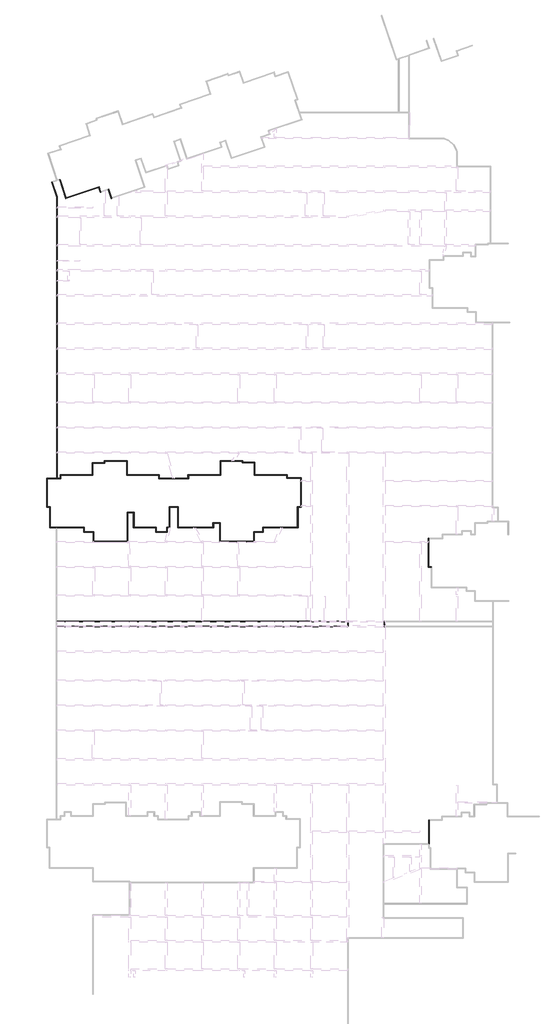
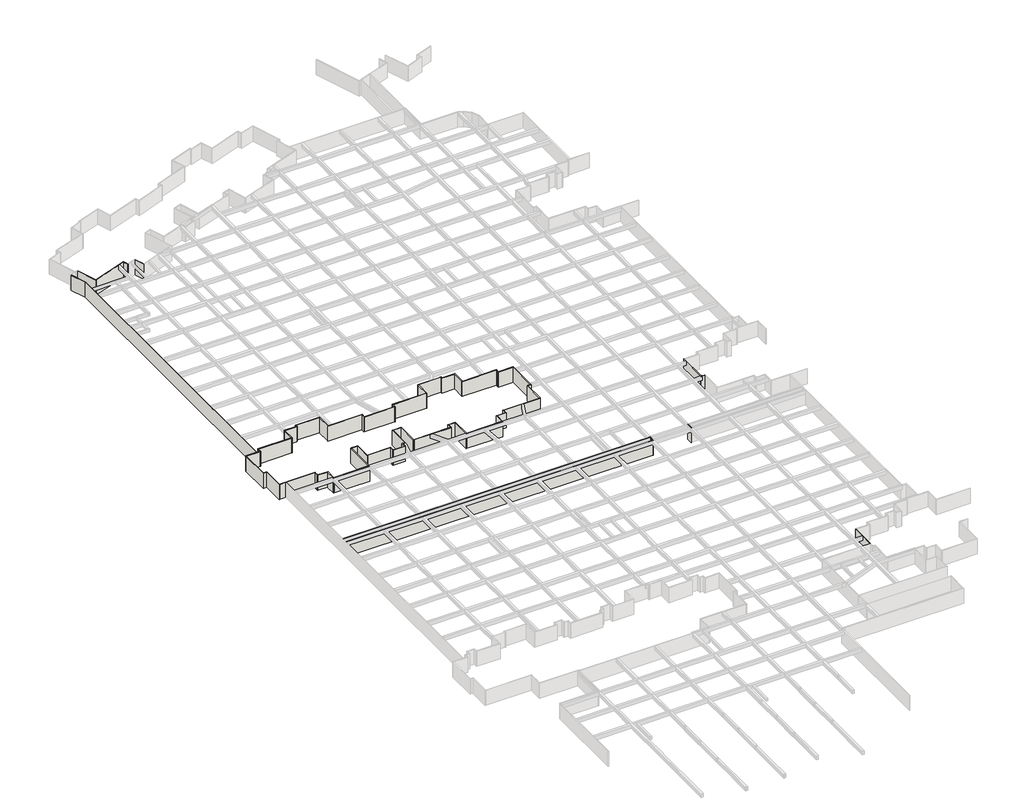
# One storey, part 3 of 14: 65 walls.
"""IFC4 building model written with IfcOpenShell, lengths in millimetres."""

import ifcopenshell
import ifcopenshell.guid

model = None  # the IFC model being written
_history = None  # IfcOwnerHistory: only IFC2X3 demands one
_inside = {}  # id of a spatial element -> (the spatial element, [elements in it])
_under = {}  # id of a project, library or spatial element -> (it, [spatial elements below it])
_declared = {}  # id of a project -> (the project, [libraries it declares])
_typed = {}  # id of a type object -> (the type object, [elements of that type])
_made_of = {}  # id of a material, layer set ... -> (it, [elements and type objects made of it])


def new_model(schema):
    """Start an empty IFC model of exactly this schema.

    Asked for "IFC4X3", IfcOpenShell would pick the latest addendum, in which some entities
    have other attributes; the version numbers below select the first issue.
    IFC2X3 requires an IfcOwnerHistory on every rooted entity: one is made here for all.
    """
    global model, _history
    if schema == "IFC4X3":
        model = ifcopenshell.file(schema_version=(4, 3, 0, 0))
    else:
        model = ifcopenshell.file(schema=schema)
    _inside.clear()
    _under.clear()
    _declared.clear()
    _typed.clear()
    _made_of.clear()
    _history = None
    if model.schema == "IFC2X3":
        org = make("IfcOrganization", Name="unknown")
        user = make(
            "IfcPersonAndOrganization",
            ThePerson=make("IfcPerson", FamilyName="unknown"),
            TheOrganization=org,
        )
        app = make(
            "IfcApplication",
            ApplicationDeveloper=org,
            Version="unknown",
            ApplicationFullName="unknown",
            ApplicationIdentifier="unknown",
        )
        _history = make(
            "IfcOwnerHistory",
            OwningUser=user,
            OwningApplication=app,
            ChangeAction="ADDED",
            CreationDate=0,
        )
    return model


def make(cls, **values):
    """One entity of the class cls with the attributes given. An attribute that is None is left unset."""
    return model.create_entity(
        cls, **{name: value for name, value in values.items() if value is not None}
    )


def rooted(cls, **values):
    """An entity with a GlobalId (a new one), such as an element, a storey or a relation."""
    return make(cls, GlobalId=ifcopenshell.guid.new(), OwnerHistory=_history, **values)


def si_unit(unit_type, name, prefix=None):
    """IfcSIUnit, for example si_unit("LENGTHUNIT", "METRE", prefix="MILLI")."""
    return make("IfcSIUnit", UnitType=unit_type, Prefix=prefix, Name=name)


def assignment(units):
    """IfcUnitAssignment: the units of a project."""
    return None if units is None else make("IfcUnitAssignment", Units=units)


def point(xyz):
    """IfcCartesianPoint."""
    return None if xyz is None else make("IfcCartesianPoint", Coordinates=xyz)


def direction(xyz):
    """IfcDirection."""
    return None if xyz is None else make("IfcDirection", DirectionRatios=xyz)


def frame(location, z_axis=None, x_axis=None):
    """IfcAxis2Placement3D, a coordinate frame: its origin and axes. An axis left out is left unset."""
    return make(
        "IfcAxis2Placement3D",
        Location=point(location),
        Axis=direction(z_axis),
        RefDirection=direction(x_axis),
    )


def origin():
    """The frame at (0, 0, 0) with its axes left unset."""
    return frame((0.0, 0.0, 0.0))


def origin_with_axes():
    """The frame at (0, 0, 0) with the z axis (0, 0, 1) and the x axis (1, 0, 0) written out."""
    return frame((0.0, 0.0, 0.0), z_axis=(0.0, 0.0, 1.0), x_axis=(1.0, 0.0, 0.0))


def place(relative_to, where):
    """IfcLocalPlacement: puts the frame where relative to a parent placement (None: the world)."""
    return make(
        "IfcLocalPlacement", PlacementRelTo=relative_to, RelativePlacement=where
    )


def context(
    kind, dimensions, precision=None, world=None, true_north=None, identifier=None
):
    """IfcGeometricRepresentationContext, for example the 3D "Model" context."""
    return make(
        "IfcGeometricRepresentationContext",
        ContextIdentifier=identifier,
        ContextType=kind,
        CoordinateSpaceDimension=dimensions,
        Precision=precision,
        WorldCoordinateSystem=world,
        TrueNorth=true_north,
    )


def project(units=None, contexts=None):
    """IfcProject with its units and contexts."""
    return rooted(
        "IfcProject",
        Name="project",
        RepresentationContexts=contexts,
        UnitsInContext=assignment(units),
    )


def spatial(cls, under=None, at=None, **own):
    """A site, building, storey or space (cls), placed at a placement, below another one or the project."""
    s = rooted(cls, ObjectPlacement=at, **own)
    if under is not None:
        _under.setdefault(under.id(), (under, []))[1].append(s)
    return s


def polyline(points):
    """IfcPolyline through the points."""
    return make("IfcPolyline", Points=[point(p) for p in points])


def outline(outer, holes=None, kind="AREA"):
    """IfcArbitraryClosedProfileDef: a profile drawn as a closed curve; with holes, ...WithVoids."""
    if holes is None:
        return make("IfcArbitraryClosedProfileDef", ProfileType=kind, OuterCurve=outer)
    return make(
        "IfcArbitraryProfileDefWithVoids",
        ProfileType=kind,
        OuterCurve=outer,
        InnerCurves=holes,
    )


def extrude(swept, where, along, depth):
    """IfcExtrudedAreaSolid: the profile swept, set in the frame where, extruded along a direction by depth."""
    return make(
        "IfcExtrudedAreaSolid",
        SweptArea=swept,
        Position=where,
        ExtrudedDirection=direction(along),
        Depth=depth,
    )


def faces_of(points, faces, orient=None, outer=None):
    """IfcFace entities. A face is a list of loops; a loop is a list of indices into points, from 0.

    orient and outer hold one flag for each loop. By default every Orientation is true, the
    first loop of a face is its IfcFaceOuterBound and the others are IfcFaceBound.
    """
    made = []
    for i, loops in enumerate(faces):
        bounds = []
        for j, loop in enumerate(loops):
            is_outer = j == 0 if outer is None else outer[i][j]
            bounds.append(
                make(
                    "IfcFaceOuterBound" if is_outer else "IfcFaceBound",
                    Bound=make("IfcPolyLoop", Polygon=[points[k] for k in loop]),
                    Orientation=True if orient is None else orient[i][j],
                )
            )
        made.append(make("IfcFace", Bounds=bounds))
    return made


def faceted_brep(points, faces, orient=None, outer=None, voids=None):
    """IfcFacetedBrep: a solid bounded by flat faces; with voids (closed shells), ...WithVoids."""
    shared = [point(p) for p in points]
    hull = make("IfcClosedShell", CfsFaces=faces_of(shared, faces, orient, outer))
    if voids is None:
        return make("IfcFacetedBrep", Outer=hull)
    return make(
        "IfcFacetedBrepWithVoids",
        Outer=hull,
        Voids=[
            make(cls, CfsFaces=faces_of(shared, fs, o, b)) for cls, fs, o, b in voids
        ],
    )


def shape(context_of_items, identifier, shape_type, items):
    """IfcShapeRepresentation: the items that make up one representation, for example the "Body"."""
    return make(
        "IfcShapeRepresentation",
        ContextOfItems=context_of_items,
        RepresentationIdentifier=identifier,
        RepresentationType=shape_type,
        Items=items,
    )


def made_of(thing, what):
    """Note that an element or type object is made of a material, layer set ...; save() writes the relation."""
    if what is not None:
        _made_of.setdefault(what.id(), (what, []))[1].append(thing)
    return thing


def element(
    cls,
    number,
    at=None,
    inside=None,
    cuts=None,
    type_object=None,
    material=None,
    context=None,
    identifier="Body",
    shape_type=None,
    held_by="IfcProductDefinitionShape",
    body=None,
    shapes=None,
    **own,
):
    """One element of the class cls, such as IfcWall. Its Tag is "e" and its number.

    at: its placement. inside: the storey or other place that contains it. cuts: it is an
    opening in that element (IfcRelVoidsElement). A single representation is given by context,
    identifier, shape_type and body (its items); several are given by shapes. held_by: the class
    of the entity that holds the representations. save() writes the other relations.
    """
    e = rooted(cls, Tag="e%d" % number, ObjectPlacement=at, **own)
    if body is not None:
        shapes = [shape(context, identifier, shape_type, body)]
    if shapes is not None:
        e.Representation = make(held_by, Representations=shapes)
    if inside is not None:
        _inside.setdefault(inside.id(), (inside, []))[1].append(e)
    if cuts is not None:
        rooted(
            "IfcRelVoidsElement", RelatingBuildingElement=cuts, RelatedOpeningElement=e
        )
    if type_object is not None:
        _typed.setdefault(type_object.id(), (type_object, []))[1].append(e)
    return made_of(e, material)


def aggregate(whole, parts):
    """IfcRelAggregates: a whole, such as a stair, and the parts it consists of."""
    return rooted("IfcRelAggregates", RelatingObject=whole, RelatedObjects=parts)


def save(model, path):
    """Write the relations noted so far, then the file.

    IfcRelAggregates (storeys below a building ...), IfcRelContainedInSpatialStructure (elements
    in a storey), IfcRelDefinesByType, IfcRelAssociatesMaterial and IfcRelDeclares: one each for
    every whole, place, type object, material and project.
    """
    for whole, parts in _under.values():
        aggregate(whole, parts)
    for where, things in _inside.values():
        rooted(
            "IfcRelContainedInSpatialStructure",
            RelatedElements=things,
            RelatingStructure=where,
        )
    for kind, things in _typed.values():
        rooted("IfcRelDefinesByType", RelatedObjects=things, RelatingType=kind)
    for what, things in _made_of.values():
        rooted("IfcRelAssociatesMaterial", RelatedObjects=things, RelatingMaterial=what)
    for by, libraries in _declared.values():
        rooted("IfcRelDeclares", RelatingContext=by, RelatedDefinitions=libraries)
    model.write(path)


model = new_model("IFC4")

# Units and contexts
model_context = context("Model", 3, world=origin())
ifc_project = project(units=[si_unit("LENGTHUNIT", "METRE", prefix="MILLI")], contexts=[model_context])

# Site, building, storey
site = spatial("IfcSite", under=ifc_project)
building = spatial("IfcBuilding", under=site)
storey = spatial("IfcBuildingStorey", under=building, Name="户型图", Elevation=0.0)

# Walls
placement = place(None, origin())
element("IfcWall", 1, ObjectType="所有墙体", at=placement, inside=storey, context=model_context, shape_type="Brep", body=[
    faceted_brep([(-593530.5298151, -30931.4697976, 0.0), (-592123.7332007, -35098.9851149, 0.0), (-592123.7332007, -35098.9851149, 3300.0), (-593530.5298151, -30931.4697976, 3300.0), (-593416.7566971, -30893.3157103, 0.0), (-593416.7566971, -30893.3157103, 3300.0), (-592048.3399682, -34947.133881, 3300.0), (-592009.9600827, -35060.8310276, 3300.0), (-592009.9600827, -35060.8310276, 0.0), (-592048.3399682, -34947.133881, 0.0)], [[[0, 1, 2, 3]], [[4, 5, 6, 7, 8, 9]], [[1, 0, 4, 9, 8]], [[3, 2, 7, 6, 5]], [[0, 3, 5, 4]], [[2, 1, 8, 7]]]),
])
element("IfcWall", 2, ObjectType="所有墙体", at=placement, inside=storey, context=model_context, shape_type="Brep", body=[
    faceted_brep([(-592009.9600827, -35060.8310276, 0.0), (-584918.2294187, -32682.6021846, 0.0), (-584804.4565249, -32644.4481725, 0.0), (-584804.4565249, -32644.4481725, 3300.0), (-584918.2294187, -32682.6021846, 3300.0), (-592009.9600827, -35060.8310276, 3300.0), (-592048.3399682, -34947.133881, 0.0), (-592048.3399682, -34947.133881, 3300.0), (-584842.610537, -32530.6752787, 3300.0), (-584842.610537, -32530.6752787, 0.0)], [[[0, 1, 2, 3, 4, 5]], [[6, 7, 8, 9]], [[2, 1, 0, 6, 9]], [[5, 4, 3, 8, 7]], [[0, 5, 7, 6]], [[3, 2, 9, 8]]]),
])
element("IfcWall", 3, ObjectType="所有墙体", at=placement, inside=storey, context=model_context, shape_type="Brep", body=[
    faceted_brep([(-584918.2294187, -32682.6021846, 0.0), (-584573.2781333, -33711.2254879, 0.0), (-584573.2781333, -33711.2254879, 3300.0), (-584918.2294187, -32682.6021846, 3300.0), (-584804.4565249, -32644.4481725, 0.0), (-584804.4565249, -32644.4481725, 3300.0), (-584497.735074, -33559.0724844, 3300.0), (-584459.5809867, -33672.8456024, 3300.0), (-584459.5809867, -33672.8456024, 0.0), (-584497.735074, -33559.0724844, 0.0)], [[[0, 1, 2, 3]], [[4, 5, 6, 7, 8, 9]], [[1, 0, 4, 9, 8]], [[3, 2, 7, 6, 5]], [[0, 3, 5, 4]], [[2, 1, 8, 7]]]),
])
element("IfcWall", 4, ObjectType="所有墙体", at=placement, inside=storey, context=model_context, shape_type="Brep", body=[
    faceted_brep([(-582772.9638867, -33103.5070288, 0.0), (-582101.3172132, -35093.2031729, 0.0), (-582101.3172132, -35093.2031729, 3300.0), (-582772.9638867, -33103.5070288, 3300.0), (-582659.2669642, -33065.1272189, 0.0), (-582659.2669642, -33065.1272189, 3300.0), (-582026.0001006, -34941.1264405, 3300.0), (-581987.6202907, -35054.823363, 3300.0), (-581987.6202907, -35054.823363, 0.0), (-582026.0001006, -34941.1264405, 0.0)], [[[0, 1, 2, 3]], [[4, 5, 6, 7, 8, 9]], [[1, 0, 4, 9, 8]], [[3, 2, 7, 6, 5]], [[0, 3, 5, 4]], [[2, 1, 8, 7]]]),
])
element("IfcWall", 5, ObjectType="所有墙体", at=placement, inside=storey, context=model_context, shape_type="SweptSolid", body=[
    extrude(outline(polyline([(-594139.2557706, -34756.12632), (-595236.3254494, -31506.1507065), (-595122.6285269, -31467.7708966), (-594019.2557706, -34736.418841), (-594139.2557706, -34756.12632)])), origin_with_axes(), (0.0, 0.0, 1.0), 3300.0),
])
element("IfcWall", 6, ObjectType="所有墙体", at=placement, inside=storey, context=model_context, shape_type="SweptSolid", body=[
    extrude(outline(polyline([(-594139.2557706, -96686.2725805), (-594139.2557706, -34756.12632), (-594019.2557706, -34736.418841), (-594019.2557706, -96686.2725805), (-594139.2557706, -96686.2725805)])), origin_with_axes(), (0.0, 0.0, 1.0), 3300.0),
])
element("IfcWall", 7, ObjectType="所有墙体", at=placement, inside=storey, context=model_context, shape_type="Brep", body=[
    faceted_brep([(-593387.5937633, -96686.2725805, 0.0), (-594019.2557706, -96686.2725805, 0.0), (-594139.2557706, -96686.2725805, 0.0), (-596357.5937917, -96686.2725805, 0.0), (-596357.5937917, -96686.2725805, 3300.0), (-594139.2557706, -96686.2725805, 3300.0), (-594019.2557706, -96686.2725805, 3300.0), (-593387.5937633, -96686.2725805, 3300.0), (-593387.5937633, -96806.2725805, 0.0), (-593387.5937633, -96806.2725805, 3300.0), (-596237.5937917, -96806.2725805, 3300.0), (-596357.5937917, -96806.2725805, 3300.0), (-596357.5937917, -96806.2725805, 0.0), (-596237.5937917, -96806.2725805, 0.0)], [[[0, 1, 2, 3, 4, 5, 6, 7]], [[8, 9, 10, 11, 12, 13]], [[3, 2, 1, 0, 8, 13, 12]], [[7, 6, 5, 4, 11, 10, 9]], [[4, 3, 12, 11]], [[0, 7, 9, 8]]]),
])
element("IfcWall", 8, ObjectType="所有墙体", at=placement, inside=storey, context=model_context, shape_type="Brep", body=[
    faceted_brep([(-596357.5937917, -96806.2725805, 0.0), (-596357.5937917, -103075.8355436, 0.0), (-596357.5937917, -103075.8355436, 3300.0), (-596357.5937917, -96806.2725805, 3300.0), (-596237.5937917, -96806.2725805, 0.0), (-596237.5937917, -96806.2725805, 3300.0), (-596237.5937917, -102955.8355436, 3300.0), (-596237.5937917, -103075.8355436, 3300.0), (-596237.5937917, -103075.8355436, 0.0), (-596237.5937917, -102955.8355436, 0.0)], [[[0, 1, 2, 3]], [[4, 5, 6, 7, 8, 9]], [[1, 0, 4, 9, 8]], [[3, 2, 7, 6, 5]], [[0, 3, 5, 4]], [[2, 1, 8, 7]]]),
])
element("IfcWall", 9, ObjectType="所有墙体", at=placement, inside=storey, context=model_context, shape_type="Brep", body=[
    faceted_brep([(-596237.5937917, -103075.8355436, 0.0), (-595657.5937933, -103075.8355436, 0.0), (-595537.5937933, -103075.8355436, 0.0), (-595537.5937933, -103075.8355436, 3300.0), (-595657.5937933, -103075.8355436, 3300.0), (-596237.5937917, -103075.8355436, 3300.0), (-596237.5937917, -102955.8355436, 0.0), (-596237.5937917, -102955.8355436, 3300.0), (-595537.5937933, -102955.8355436, 3300.0), (-595537.5937933, -102955.8355436, 0.0)], [[[0, 1, 2, 3, 4, 5]], [[6, 7, 8, 9]], [[2, 1, 0, 6, 9]], [[5, 4, 3, 8, 7]], [[0, 5, 7, 6]], [[3, 2, 9, 8]]]),
])
element("IfcWall", 10, ObjectType="所有墙体", at=placement, inside=storey, context=model_context, shape_type="Brep", body=[
    faceted_brep([(-595657.5937933, -103075.8355436, 0.0), (-595657.5937933, -107575.8355437, 0.0), (-595657.5937933, -107575.8355437, 3300.0), (-595657.5937933, -103075.8355436, 3300.0), (-595537.5937933, -103075.8355436, 0.0), (-595537.5937933, -103075.8355436, 3300.0), (-595537.5937933, -107455.8355437, 3300.0), (-595537.5937933, -107575.8355437, 3300.0), (-595537.5937933, -107575.8355437, 0.0), (-595537.5937933, -107455.8355437, 0.0)], [[[0, 1, 2, 3]], [[4, 5, 6, 7, 8, 9]], [[1, 0, 4, 9, 8]], [[3, 2, 7, 6, 5]], [[0, 3, 5, 4]], [[2, 1, 8, 7]]]),
])
element("IfcWall", 11, ObjectType="所有墙体", at=placement, inside=storey, context=model_context, shape_type="Brep", body=[
    faceted_brep([(-595537.5937933, -107575.8355437, 0.0), (-594257.5937933, -107575.8355437, 0.0), (-594137.5937933, -107575.8355437, 0.0), (-588182.5937843, -107575.8355437, 0.0), (-588062.5937843, -107575.8355437, 0.0), (-588062.5937843, -107575.8355437, 3300.0), (-588182.5937843, -107575.8355437, 3300.0), (-594137.5937933, -107575.8355437, 3300.0), (-594257.5937933, -107575.8355437, 3300.0), (-595537.5937933, -107575.8355437, 3300.0), (-595537.5937933, -107455.8355437, 0.0), (-595537.5937933, -107455.8355437, 3300.0), (-588062.5937843, -107455.8355437, 3300.0), (-588062.5937843, -107455.8355437, 0.0)], [[[0, 1, 2, 3, 4, 5, 6, 7, 8, 9]], [[10, 11, 12, 13]], [[4, 3, 2, 1, 0, 10, 13]], [[9, 8, 7, 6, 5, 12, 11]], [[0, 9, 11, 10]], [[5, 4, 13, 12]]]),
])
element("IfcWall", 12, ObjectType="所有墙体", at=placement, inside=storey, context=model_context, shape_type="Brep", body=[
    faceted_brep([(-588182.5937843, -107575.8355437, 0.0), (-588182.5937843, -108525.8355399, 0.0), (-588182.5937843, -108525.8355399, 3300.0), (-588182.5937843, -107575.8355437, 3300.0), (-588062.5937843, -107575.8355437, 0.0), (-588062.5937843, -107575.8355437, 3300.0), (-588062.5937843, -108405.8355399, 3300.0), (-588062.5937843, -108525.8355399, 3300.0), (-588062.5937843, -108525.8355399, 0.0), (-588062.5937843, -108405.8355399, 0.0)], [[[0, 1, 2, 3]], [[4, 5, 6, 7, 8, 9]], [[1, 0, 4, 9, 8]], [[3, 2, 7, 6, 5]], [[0, 3, 5, 4]], [[2, 1, 8, 7]]]),
])
element("IfcWall", 13, ObjectType="所有墙体", at=placement, inside=storey, context=model_context, shape_type="Brep", body=[
    faceted_brep([(-588062.5937843, -108525.8355399, 0.0), (-586077.6529954, -108525.8355399, 0.0), (-585957.6529954, -108525.8355399, 0.0), (-585957.6529954, -108525.8355399, 3300.0), (-586077.6529954, -108525.8355399, 3300.0), (-588062.5937843, -108525.8355399, 3300.0), (-588062.5937843, -108405.8355399, 0.0), (-588062.5937843, -108405.8355399, 3300.0), (-585957.6529954, -108405.8355399, 3300.0), (-585957.6529954, -108405.8355399, 0.0)], [[[0, 1, 2, 3, 4, 5]], [[6, 7, 8, 9]], [[2, 1, 0, 6, 9]], [[5, 4, 3, 8, 7]], [[0, 5, 7, 6]], [[3, 2, 9, 8]]]),
])
element("IfcWall", 14, ObjectType="所有墙体", at=placement, inside=storey, context=model_context, shape_type="Brep", body=[
    faceted_brep([(-586077.6529954, -108525.8355399, 0.0), (-586077.6529954, -110675.8355352, 0.0), (-586077.6529954, -110675.8355352, 2500.0), (-586077.6529954, -110675.8355352, 3300.0), (-586077.6529954, -110459.4327531, 3300.0), (-586077.6529954, -108525.8355399, 3300.0), (-585957.6529954, -108525.8355399, 0.0), (-585957.6529954, -108525.8355399, 3300.0), (-585957.6529954, -110459.4327531, 3300.0), (-585957.6529954, -110555.8355352, 3300.0), (-585957.6529954, -110675.8355352, 3300.0), (-585957.6529954, -110675.8355352, 0.0), (-585957.6529954, -110555.8355352, 0.0)], [[[0, 1, 2, 3, 4, 5]], [[6, 7, 8, 9, 10, 11, 12]], [[1, 0, 6, 12, 11]], [[5, 4, 3, 10, 9, 8, 7]], [[0, 5, 7, 6]], [[3, 2, 1, 11, 10]]]),
])
element("IfcWall", 15, ObjectType="所有墙体", at=placement, inside=storey, context=model_context, shape_type="Brep", body=[
    faceted_brep([(-585957.6529954, -110675.8355352, 0.0), (-578537.5937894, -110675.8355352, 0.0), (-578537.5937894, -110675.8355352, 2500.0), (-578537.5937894, -110675.8355352, 3300.0), (-585957.6529954, -110675.8355352, 3300.0), (-585957.6529954, -110555.8355352, 0.0), (-585957.6529954, -110555.8355352, 2500.0), (-585957.6529954, -110555.8355352, 3300.0), (-578657.5937894, -110555.8355352, 3300.0), (-578537.5937894, -110555.8355352, 3300.0), (-578537.5937894, -110555.8355352, 0.0), (-578657.5937894, -110555.8355352, 0.0)], [[[0, 1, 2, 3, 4]], [[5, 6, 7, 8, 9, 10, 11]], [[1, 0, 5, 11, 10]], [[4, 3, 9, 8, 7]], [[0, 4, 7, 6, 5]], [[3, 2, 1, 10, 9]]]),
])
element("IfcWall", 16, ObjectType="所有墙体", at=placement, inside=storey, context=model_context, shape_type="Brep", body=[
    faceted_brep([(-578537.5937894, -110555.8355352, 0.0), (-578537.5937894, -104200.8355452, 0.0), (-578537.5937894, -104080.8355452, 0.0), (-578537.5937894, -104080.8355452, 3300.0), (-578537.5937894, -104200.8355452, 3300.0), (-578537.5937894, -110459.4327531, 3300.0), (-578537.5937894, -110555.8355352, 3300.0), (-578657.5937894, -110555.8355352, 0.0), (-578657.5937894, -110555.8355352, 2500.0), (-578657.5937894, -110555.8355352, 3300.0), (-578657.5937894, -110459.4327531, 3300.0), (-578657.5937894, -104080.8355452, 3300.0), (-578657.5937894, -104080.8355452, 0.0)], [[[0, 1, 2, 3, 4, 5, 6]], [[7, 8, 9, 10, 11, 12]], [[2, 1, 0, 7, 12]], [[6, 5, 4, 3, 11, 10, 9]], [[0, 6, 9, 8, 7]], [[3, 2, 12, 11]]]),
])
element("IfcWall", 17, ObjectType="所有墙体", at=placement, inside=storey, context=model_context, shape_type="Brep", body=[
    faceted_brep([(-578537.5937894, -104200.8355452, 0.0), (-577257.5937775, -104200.8355452, 0.0), (-577137.5937775, -104200.8355452, 0.0), (-577137.5937775, -104200.8355452, 3300.0), (-577257.5937775, -104200.8355452, 3300.0), (-578537.5937894, -104200.8355452, 3300.0), (-578537.5937894, -104080.8355452, 0.0), (-578537.5937894, -104080.8355452, 3300.0), (-577137.5937775, -104080.8355452, 3300.0), (-577137.5937775, -104080.8355452, 0.0)], [[[0, 1, 2, 3, 4, 5]], [[6, 7, 8, 9]], [[2, 1, 0, 6, 9]], [[5, 4, 3, 8, 7]], [[0, 5, 7, 6]], [[3, 2, 9, 8]]]),
])
element("IfcWall", 18, ObjectType="所有墙体", at=placement, inside=storey, context=model_context, shape_type="Brep", body=[
    faceted_brep([(-577257.5937775, -104200.8355452, 0.0), (-577257.5937775, -107575.8355437, 0.0), (-577257.5937775, -107575.8355437, 3300.0), (-577257.5937775, -104200.8355452, 3300.0), (-577137.5937775, -104200.8355452, 0.0), (-577137.5937775, -104200.8355452, 3300.0), (-577137.5937775, -107455.8355437, 3300.0), (-577137.5937775, -107575.8355437, 3300.0), (-577137.5937775, -107575.8355437, 0.0), (-577137.5937775, -107455.8355437, 0.0)], [[[0, 1, 2, 3]], [[4, 5, 6, 7, 8, 9]], [[1, 0, 4, 9, 8]], [[3, 2, 7, 6, 5]], [[0, 3, 5, 4]], [[2, 1, 8, 7]]]),
])
element("IfcWall", 19, ObjectType="所有墙体", at=placement, inside=storey, context=model_context, shape_type="Brep", body=[
    faceted_brep([(-577137.5937775, -107575.8355437, 0.0), (-572407.593776, -107575.8355437, 0.0), (-572287.593776, -107575.8355437, 0.0), (-572287.593776, -107575.8355437, 3300.0), (-572407.593776, -107575.8355437, 3300.0), (-577137.5937775, -107575.8355437, 3300.0), (-577137.5937775, -107455.8355437, 0.0), (-577137.5937775, -107455.8355437, 3300.0), (-572287.593776, -107455.8355437, 3300.0), (-572287.593776, -107455.8355437, 0.0)], [[[0, 1, 2, 3, 4, 5]], [[6, 7, 8, 9]], [[2, 1, 0, 6, 9]], [[5, 4, 3, 8, 7]], [[0, 5, 7, 6]], [[3, 2, 9, 8]]]),
])
element("IfcWall", 20, ObjectType="所有墙体", at=placement, inside=storey, context=model_context, shape_type="Brep", body=[
    faceted_brep([(-572407.593776, -107575.8355437, 0.0), (-572407.593776, -108525.8355399, 0.0), (-572407.593776, -108525.8355399, 3300.0), (-572407.593776, -107575.8355437, 3300.0), (-572287.593776, -107575.8355437, 0.0), (-572287.593776, -107575.8355437, 3300.0), (-572287.593776, -108405.8355399, 3300.0), (-572287.593776, -108525.8355399, 3300.0), (-572287.593776, -108525.8355399, 0.0), (-572287.593776, -108405.8355399, 0.0)], [[[0, 1, 2, 3]], [[4, 5, 6, 7, 8, 9]], [[1, 0, 4, 9, 8]], [[3, 2, 7, 6, 5]], [[0, 3, 5, 4]], [[2, 1, 8, 7]]]),
])
element("IfcWall", 21, ObjectType="所有墙体", at=placement, inside=storey, context=model_context, shape_type="Brep", body=[
    faceted_brep([(-572287.593776, -108525.8355399, 0.0), (-569787.5937802, -108525.8355399, 0.0), (-569787.5937802, -108525.8355399, 3300.0), (-572287.593776, -108525.8355399, 3300.0), (-572287.593776, -108405.8355399, 0.0), (-572287.593776, -108405.8355399, 3300.0), (-569907.5937802, -108405.8355399, 3300.0), (-569787.5937802, -108405.8355399, 3300.0), (-569787.5937802, -108405.8355399, 0.0), (-569907.5937802, -108405.8355399, 0.0)], [[[0, 1, 2, 3]], [[4, 5, 6, 7, 8, 9]], [[1, 0, 4, 9, 8]], [[3, 2, 7, 6, 5]], [[0, 3, 5, 4]], [[2, 1, 8, 7]]]),
])
element("IfcWall", 22, ObjectType="所有墙体", at=placement, inside=storey, context=model_context, shape_type="Brep", body=[
    faceted_brep([(-569787.5937802, -108405.8355399, 0.0), (-569787.5937802, -107575.8355437, 0.0), (-569787.5937802, -107455.8355437, 0.0), (-569787.5937802, -107455.8355437, 3300.0), (-569787.5937802, -107575.8355437, 3300.0), (-569787.5937802, -108405.8355399, 3300.0), (-569907.5937802, -108405.8355399, 0.0), (-569907.5937802, -108405.8355399, 3300.0), (-569907.5937802, -107455.8355437, 3300.0), (-569907.5937802, -107455.8355437, 0.0)], [[[0, 1, 2, 3, 4, 5]], [[6, 7, 8, 9]], [[2, 1, 0, 6, 9]], [[5, 4, 3, 8, 7]], [[0, 5, 7, 6]], [[3, 2, 9, 8]]]),
])
element("IfcWall", 23, ObjectType="所有墙体", at=placement, inside=storey, context=model_context, shape_type="Brep", body=[
    faceted_brep([(-569787.5937802, -107575.8355437, 0.0), (-569237.5937855, -107575.8355437, 0.0), (-569237.5937855, -107575.8355437, 3300.0), (-569787.5937802, -107575.8355437, 3300.0), (-569787.5937802, -107455.8355437, 0.0), (-569787.5937802, -107455.8355437, 3300.0), (-569357.5937855, -107455.8355437, 3300.0), (-569237.5937855, -107455.8355437, 3300.0), (-569237.5937855, -107455.8355437, 0.0), (-569357.5937855, -107455.8355437, 0.0)], [[[0, 1, 2, 3]], [[4, 5, 6, 7, 8, 9]], [[1, 0, 4, 9, 8]], [[3, 2, 7, 6, 5]], [[0, 3, 5, 4]], [[2, 1, 8, 7]]]),
])
element("IfcWall", 24, ObjectType="所有墙体", at=placement, inside=storey, context=model_context, shape_type="Brep", body=[
    faceted_brep([(-569237.5937855, -107455.8355437, 0.0), (-569237.5937855, -103075.8355436, 0.0), (-569237.5937855, -102955.8355436, 0.0), (-569237.5937855, -102955.8355436, 3300.0), (-569237.5937855, -103075.8355436, 3300.0), (-569237.5937855, -107455.8355437, 3300.0), (-569357.5937855, -107455.8355437, 0.0), (-569357.5937855, -107455.8355437, 3300.0), (-569357.5937855, -102955.8355436, 3300.0), (-569357.5937855, -102955.8355436, 0.0)], [[[0, 1, 2, 3, 4, 5]], [[6, 7, 8, 9]], [[2, 1, 0, 6, 9]], [[5, 4, 3, 8, 7]], [[0, 5, 7, 6]], [[3, 2, 9, 8]]]),
])
element("IfcWall", 25, ObjectType="所有墙体", at=placement, inside=storey, context=model_context, shape_type="Brep", body=[
    faceted_brep([(-569237.5937855, -103075.8355436, 0.0), (-567557.5937887, -103075.8355436, 0.0), (-567437.5937887, -103075.8355436, 0.0), (-567437.5937887, -103075.8355436, 3300.0), (-567557.5937887, -103075.8355436, 3300.0), (-569237.5937855, -103075.8355436, 3300.0), (-569237.5937855, -102955.8355436, 0.0), (-569237.5937855, -102955.8355436, 3300.0), (-567437.5937887, -102955.8355436, 3300.0), (-567437.5937887, -102955.8355436, 0.0)], [[[0, 1, 2, 3, 4, 5]], [[6, 7, 8, 9]], [[2, 1, 0, 6, 9]], [[5, 4, 3, 8, 7]], [[0, 5, 7, 6]], [[3, 2, 9, 8]]]),
])
element("IfcWall", 26, ObjectType="所有墙体", at=placement, inside=storey, context=model_context, shape_type="Brep", body=[
    faceted_brep([(-567557.5937887, -103075.8355436, 0.0), (-567557.5937887, -107575.8355437, 0.0), (-567557.5937887, -107575.8355437, 3300.0), (-567557.5937887, -103075.8355436, 3300.0), (-567437.5937887, -103075.8355436, 0.0), (-567437.5937887, -103075.8355436, 3300.0), (-567437.5937887, -107455.8355437, 3300.0), (-567437.5937887, -107575.8355437, 3300.0), (-567437.5937887, -107575.8355437, 0.0), (-567437.5937887, -107455.8355437, 0.0)], [[[0, 1, 2, 3]], [[4, 5, 6, 7, 8, 9]], [[1, 0, 4, 9, 8]], [[3, 2, 7, 6, 5]], [[0, 3, 5, 4]], [[2, 1, 8, 7]]]),
])
element("IfcWall", 27, ObjectType="所有墙体", at=placement, inside=storey, context=model_context, shape_type="Brep", body=[
    faceted_brep([(-567437.5937887, -107575.8355437, 0.0), (-559637.5937886, -107575.8355437, 0.0), (-559637.5937886, -107575.8355437, 3300.0), (-567437.5937887, -107575.8355437, 3300.0), (-567437.5937887, -107455.8355437, 0.0), (-567437.5937887, -107455.8355437, 3300.0), (-559757.5937886, -107455.8355437, 3300.0), (-559637.5937886, -107455.8355437, 3300.0), (-559637.5937886, -107455.8355437, 0.0), (-559757.5937886, -107455.8355437, 0.0)], [[[0, 1, 2, 3]], [[4, 5, 6, 7, 8, 9]], [[1, 0, 4, 9, 8]], [[3, 2, 7, 6, 5]], [[0, 3, 5, 4]], [[2, 1, 8, 7]]]),
])
element("IfcWall", 28, ObjectType="所有墙体", at=placement, inside=storey, context=model_context, shape_type="Brep", body=[
    faceted_brep([(-559637.5937886, -107455.8355437, 0.0), (-559637.5937886, -106575.8355437, 0.0), (-559637.5937886, -106455.8355437, 0.0), (-559637.5937886, -106455.8355437, 3300.0), (-559637.5937886, -106575.8355437, 3300.0), (-559637.5937886, -107455.8355437, 3300.0), (-559757.5937886, -107455.8355437, 0.0), (-559757.5937886, -107455.8355437, 3300.0), (-559757.5937886, -106455.8355437, 3300.0), (-559757.5937886, -106455.8355437, 0.0)], [[[0, 1, 2, 3, 4, 5]], [[6, 7, 8, 9]], [[2, 1, 0, 6, 9]], [[5, 4, 3, 8, 7]], [[0, 5, 7, 6]], [[3, 2, 9, 8]]]),
])
element("IfcWall", 29, ObjectType="所有墙体", at=placement, inside=storey, context=model_context, shape_type="Brep", body=[
    faceted_brep([(-559637.5937886, -106575.8355437, 0.0), (-558257.5932626, -106575.8355437, 0.0), (-558137.5932626, -106575.8355437, 0.0), (-558137.5932626, -106575.8355437, 3300.0), (-558257.5932626, -106575.8355437, 3300.0), (-559637.5937886, -106575.8355437, 3300.0), (-559637.5937886, -106455.8355437, 0.0), (-559637.5937886, -106455.8355437, 3300.0), (-558137.5932626, -106455.8355437, 3300.0), (-558137.5932626, -106455.8355437, 0.0)], [[[0, 1, 2, 3, 4, 5]], [[6, 7, 8, 9]], [[2, 1, 0, 6, 9]], [[5, 4, 3, 8, 7]], [[0, 5, 7, 6]], [[3, 2, 9, 8]]]),
])
element("IfcWall", 30, ObjectType="所有墙体", at=placement, inside=storey, context=model_context, shape_type="Brep", body=[
    faceted_brep([(-558257.5932626, -106575.8355437, 0.0), (-558257.5932626, -110575.8355372, 0.0), (-558257.5932626, -110575.8355372, 2500.0), (-558257.5932626, -110575.8355372, 3300.0), (-558257.5932626, -110459.4327531, 3300.0), (-558257.5932626, -106575.8355437, 3300.0), (-558137.5932626, -106575.8355437, 0.0), (-558137.5932626, -106575.8355437, 3300.0), (-558137.5932626, -110455.8355372, 3300.0), (-558137.5932626, -110575.8355372, 3300.0), (-558137.5932626, -110575.8355372, 0.0), (-558137.5932626, -110455.8355372, 0.0)], [[[0, 1, 2, 3, 4, 5]], [[6, 7, 8, 9, 10, 11]], [[1, 0, 6, 11, 10]], [[5, 4, 3, 9, 8, 7]], [[0, 5, 7, 6]], [[3, 2, 1, 10, 9]]]),
])
element("IfcWall", 31, ObjectType="所有墙体", at=placement, inside=storey, context=model_context, shape_type="Brep", body=[
    faceted_brep([(-558137.5932626, -110575.8355372, 0.0), (-550637.5937889, -110575.8355372, 0.0), (-550637.5937889, -110575.8355372, 2500.0), (-550637.5937889, -110575.8355372, 3300.0), (-558137.5932626, -110575.8355372, 3300.0), (-558137.5932626, -110455.8355372, 0.0), (-558137.5932626, -110455.8355372, 3300.0), (-550757.5937889, -110455.8355372, 3300.0), (-550637.5937889, -110455.8355372, 3300.0), (-550637.5937889, -110455.8355372, 0.0), (-550757.5937889, -110455.8355372, 0.0), (-550637.5937889, -110459.4327531, 3300.0)], [[[0, 1, 2, 3, 4]], [[5, 6, 7, 8, 9, 10]], [[1, 0, 5, 10, 9]], [[4, 3, 11, 8, 7, 6]], [[0, 4, 6, 5]], [[3, 2, 1, 9, 8, 11]]]),
])
element("IfcWall", 32, ObjectType="所有墙体", at=placement, inside=storey, context=model_context, shape_type="Brep", body=[
    faceted_brep([(-550637.5937889, -110455.8355372, 0.0), (-550637.5937889, -108525.8355399, 0.0), (-550637.5937889, -108405.8355399, 0.0), (-550637.5937889, -108405.8355399, 3300.0), (-550637.5937889, -108525.8355399, 3300.0), (-550637.5937889, -110455.8355372, 3300.0), (-550757.5937889, -110455.8355372, 0.0), (-550757.5937889, -110455.8355372, 3300.0), (-550757.5937889, -108405.8355399, 3300.0), (-550757.5937889, -108405.8355399, 0.0)], [[[0, 1, 2, 3, 4, 5]], [[6, 7, 8, 9]], [[2, 1, 0, 6, 9]], [[5, 4, 3, 8, 7]], [[0, 5, 7, 6]], [[3, 2, 9, 8]]]),
])
element("IfcWall", 33, ObjectType="所有墙体", at=placement, inside=storey, context=model_context, shape_type="Brep", body=[
    faceted_brep([(-550637.5937889, -108525.8355399, 0.0), (-548737.5937889, -108525.8355399, 0.0), (-548737.5937889, -108525.8355399, 3300.0), (-550637.5937889, -108525.8355399, 3300.0), (-550637.5937889, -108405.8355399, 0.0), (-550637.5937889, -108405.8355399, 3300.0), (-548857.5937889, -108405.8355399, 3300.0), (-548737.5937889, -108405.8355399, 3300.0), (-548737.5937889, -108405.8355399, 0.0), (-548857.5937889, -108405.8355399, 0.0)], [[[0, 1, 2, 3]], [[4, 5, 6, 7, 8, 9]], [[1, 0, 4, 9, 8]], [[3, 2, 7, 6, 5]], [[0, 3, 5, 4]], [[2, 1, 8, 7]]]),
])
element("IfcWall", 34, ObjectType="所有墙体", at=placement, inside=storey, context=model_context, shape_type="Brep", body=[
    faceted_brep([(-548737.5937889, -108405.8355399, 0.0), (-548737.5937889, -107575.8355437, 0.0), (-548737.5937889, -107455.8355437, 0.0), (-548737.5937889, -107455.8355437, 3300.0), (-548737.5937889, -107575.8355437, 3300.0), (-548737.5937889, -108405.8355399, 3300.0), (-548857.5937889, -108405.8355399, 0.0), (-548857.5937889, -108405.8355399, 3300.0), (-548857.5937889, -107455.8355437, 3300.0), (-548857.5937889, -107455.8355437, 0.0)], [[[0, 1, 2, 3, 4, 5]], [[6, 7, 8, 9]], [[2, 1, 0, 6, 9]], [[5, 4, 3, 8, 7]], [[0, 5, 7, 6]], [[3, 2, 9, 8]]]),
])
element("IfcWall", 35, ObjectType="所有墙体", at=placement, inside=storey, context=model_context, shape_type="Brep", body=[
    faceted_brep([(-548737.5937889, -107575.8355437, 0.0), (-541037.5937889, -107575.8355437, 0.0), (-541037.5937889, -107575.8355437, 3300.0), (-548737.5937889, -107575.8355437, 3300.0), (-548737.5937889, -107455.8355437, 0.0), (-548737.5937889, -107455.8355437, 3300.0), (-541157.5937889, -107455.8355437, 3300.0), (-541037.5937889, -107455.8355437, 3300.0), (-541037.5937889, -107455.8355437, 0.0), (-541157.5937889, -107455.8355437, 0.0)], [[[0, 1, 2, 3]], [[4, 5, 6, 7, 8, 9]], [[1, 0, 4, 9, 8]], [[3, 2, 7, 6, 5]], [[0, 3, 5, 4]], [[2, 1, 8, 7]]]),
])
element("IfcWall", 36, ObjectType="所有墙体", at=placement, inside=storey, context=model_context, shape_type="Brep", body=[
    faceted_brep([(-541037.5937889, -107455.8355437, 0.0), (-541037.5937889, -103075.8355437, 0.0), (-541037.5937889, -102955.8355437, 0.0), (-541037.5937889, -102955.8355437, 3300.0), (-541037.5937889, -103075.8355437, 3300.0), (-541037.5937889, -107455.8355437, 3300.0), (-541157.5937889, -107455.8355437, 0.0), (-541157.5937889, -107455.8355437, 3300.0), (-541157.5937889, -102955.8355437, 3300.0), (-541157.5937889, -102955.8355437, 0.0)], [[[0, 1, 2, 3, 4, 5]], [[6, 7, 8, 9]], [[2, 1, 0, 6, 9]], [[5, 4, 3, 8, 7]], [[0, 5, 7, 6]], [[3, 2, 9, 8]]]),
])
element("IfcWall", 37, ObjectType="所有墙体", at=placement, inside=storey, context=model_context, shape_type="Brep", body=[
    faceted_brep([(-541037.5937889, -103075.8355437, 0.0), (-540337.593755, -103075.8355437, 0.0), (-540337.593755, -103075.8355437, 3300.0), (-541037.5937889, -103075.8355437, 3300.0), (-541037.5937889, -102955.8355437, 0.0), (-541037.5937889, -102955.8355437, 3300.0), (-540457.593755, -102955.8355437, 3300.0), (-540337.593755, -102955.8355437, 3300.0), (-540337.593755, -102955.8355437, 0.0), (-540457.593755, -102955.8355437, 0.0), (-540337.593755, -102959.4327531, 3300.0)], [[[0, 1, 2, 3]], [[4, 5, 6, 7, 8, 9]], [[1, 0, 4, 9, 8]], [[3, 2, 10, 7, 6, 5]], [[0, 3, 5, 4]], [[2, 1, 8, 7, 10]]]),
])
element("IfcWall", 38, ObjectType="所有墙体", at=placement, inside=storey, context=model_context, shape_type="Brep", body=[
    faceted_brep([(-540337.593755, -102955.8355437, 0.0), (-540337.593755, -96555.8355589, 0.0), (-540337.593755, -96555.8355589, 3300.0), (-540337.593755, -102955.8355437, 3300.0), (-540457.593755, -102955.8355437, 0.0), (-540457.593755, -102955.8355437, 3300.0), (-540457.593755, -96675.8355589, 3300.0), (-540457.593755, -96555.8355589, 3300.0), (-540457.593755, -96555.8355589, 0.0), (-540457.593755, -96675.8355589, 0.0)], [[[0, 1, 2, 3]], [[4, 5, 6, 7, 8, 9]], [[1, 0, 4, 9, 8]], [[3, 2, 7, 6, 5]], [[0, 3, 5, 4]], [[2, 1, 8, 7]]]),
])
element("IfcWall", 39, ObjectType="所有墙体", at=placement, inside=storey, context=model_context, shape_type="Brep", body=[
    faceted_brep([(-540457.593755, -96555.8355589, 0.0), (-543437.5937842, -96555.8355589, 0.0), (-543557.5937842, -96555.8355589, 0.0), (-543557.5937842, -96555.8355589, 3300.0), (-543437.5937842, -96555.8355589, 3300.0), (-540457.593755, -96555.8355589, 3300.0), (-540457.593755, -96675.8355589, 0.0), (-540457.593755, -96675.8355589, 3300.0), (-543557.5937842, -96675.8355589, 3300.0), (-543557.5937842, -96675.8355589, 0.0)], [[[0, 1, 2, 3, 4, 5]], [[6, 7, 8, 9]], [[2, 1, 0, 6, 9]], [[5, 4, 3, 8, 7]], [[0, 5, 7, 6]], [[3, 2, 9, 8]]]),
])
element("IfcWall", 40, ObjectType="所有墙体", at=placement, inside=storey, context=model_context, shape_type="Brep", body=[
    faceted_brep([(-543437.5937842, -96555.8355589, 0.0), (-543437.5937842, -95855.8355501, 0.0), (-543437.5937842, -95855.8355501, 3300.0), (-543437.5937842, -96555.8355589, 3300.0), (-543557.5937842, -96555.8355589, 0.0), (-543557.5937842, -96555.8355589, 3300.0), (-543557.5937842, -95975.8355501, 3300.0), (-543557.5937842, -95855.8355501, 3300.0), (-543557.5937842, -95855.8355501, 0.0), (-543557.5937842, -95975.8355501, 0.0)], [[[0, 1, 2, 3]], [[4, 5, 6, 7, 8, 9]], [[1, 0, 4, 9, 8]], [[3, 2, 7, 6, 5]], [[0, 3, 5, 4]], [[2, 1, 8, 7]]]),
])
element("IfcWall", 41, ObjectType="所有墙体", at=placement, inside=storey, context=model_context, shape_type="Brep", body=[
    faceted_brep([(-543557.5937842, -95855.8355501, 0.0), (-550537.5937827, -95855.8355501, 0.0), (-550657.5937827, -95855.8355501, 0.0), (-550657.5937827, -95855.8355501, 3300.0), (-550537.5937827, -95855.8355501, 3300.0), (-543557.5937842, -95855.8355501, 3300.0), (-543557.5937842, -95975.8355501, 0.0), (-543557.5937842, -95975.8355501, 3300.0), (-550657.5937827, -95975.8355501, 3300.0), (-550657.5937827, -95975.8355501, 0.0)], [[[0, 1, 2, 3, 4, 5]], [[6, 7, 8, 9]], [[2, 1, 0, 6, 9]], [[5, 4, 3, 8, 7]], [[0, 5, 7, 6]], [[3, 2, 9, 8]]]),
])
element("IfcWall", 42, ObjectType="所有墙体", at=placement, inside=storey, context=model_context, shape_type="Brep", body=[
    faceted_brep([(-550537.5937827, -95855.8355501, 0.0), (-550537.5937827, -93105.8355875, 0.0), (-550537.5937827, -93105.8355875, 3300.0), (-550537.5937827, -95855.8355501, 3300.0), (-550657.5937827, -95855.8355501, 0.0), (-550657.5937827, -95855.8355501, 3300.0), (-550657.5937827, -93225.8355875, 3300.0), (-550657.5937827, -93105.8355875, 3300.0), (-550657.5937827, -93105.8355875, 0.0), (-550657.5937827, -93225.8355875, 0.0)], [[[0, 1, 2, 3]], [[4, 5, 6, 7, 8, 9]], [[1, 0, 4, 9, 8]], [[3, 2, 7, 6, 5]], [[0, 3, 5, 4]], [[2, 1, 8, 7]]]),
])
element("IfcWall", 43, ObjectType="所有墙体", at=placement, inside=storey, context=model_context, shape_type="Brep", body=[
    faceted_brep([(-550657.5937827, -93105.8355875, 0.0), (-553237.5937827, -93105.8355875, 0.0), (-553357.5937827, -93105.8355875, 0.0), (-553357.5937827, -93105.8355875, 3300.0), (-553237.5937827, -93105.8355875, 3300.0), (-550657.5937827, -93105.8355875, 3300.0), (-550657.5937827, -93225.8355875, 0.0), (-550657.5937827, -93225.8355875, 3300.0), (-553357.5937827, -93225.8355875, 3300.0), (-553357.5937827, -93225.8355875, 0.0)], [[[0, 1, 2, 3, 4, 5]], [[6, 7, 8, 9]], [[2, 1, 0, 6, 9]], [[5, 4, 3, 8, 7]], [[0, 5, 7, 6]], [[3, 2, 9, 8]]]),
])
element("IfcWall", 44, ObjectType="所有墙体", at=placement, inside=storey, context=model_context, shape_type="Brep", body=[
    faceted_brep([(-553237.5937827, -93105.8355875, 0.0), (-553237.5937827, -92805.8355834, 0.0), (-553237.5937827, -92805.8355834, 3300.0), (-553237.5937827, -93105.8355875, 3300.0), (-553357.5937827, -93105.8355875, 0.0), (-553357.5937827, -93105.8355875, 3300.0), (-553357.5937827, -92925.8355834, 3300.0), (-553357.5937827, -92805.8355834, 3300.0), (-553357.5937827, -92805.8355834, 0.0), (-553357.5937827, -92925.8355834, 0.0)], [[[0, 1, 2, 3]], [[4, 5, 6, 7, 8, 9]], [[1, 0, 4, 9, 8]], [[3, 2, 7, 6, 5]], [[0, 3, 5, 4]], [[2, 1, 8, 7]]]),
])
element("IfcWall", 45, ObjectType="所有墙体", at=placement, inside=storey, context=model_context, shape_type="Brep", body=[
    faceted_brep([(-553357.5937827, -92805.8355834, 0.0), (-558157.5937827, -92805.8355834, 0.0), (-558157.5937827, -92805.8355834, 3300.0), (-553357.5937827, -92805.8355834, 3300.0), (-553357.5937827, -92925.8355834, 0.0), (-553357.5937827, -92925.8355834, 3300.0), (-558037.5937827, -92925.8355834, 3300.0), (-558157.5937827, -92925.8355834, 3300.0), (-558157.5937827, -92925.8355834, 0.0), (-558037.5937827, -92925.8355834, 0.0)], [[[0, 1, 2, 3]], [[4, 5, 6, 7, 8, 9]], [[1, 0, 4, 9, 8]], [[3, 2, 7, 6, 5]], [[0, 3, 5, 4]], [[2, 1, 8, 7]]]),
])
element("IfcWall", 46, ObjectType="所有墙体", at=placement, inside=storey, context=model_context, shape_type="Brep", body=[
    faceted_brep([(-558157.5937827, -92925.8355834, 0.0), (-558157.5937827, -95855.8355501, 0.0), (-558157.5937827, -95975.8355501, 0.0), (-558157.5937827, -95975.8355501, 3300.0), (-558157.5937827, -95855.8355501, 3300.0), (-558157.5937827, -92925.8355834, 3300.0), (-558037.5937827, -92925.8355834, 0.0), (-558037.5937827, -92925.8355834, 3300.0), (-558037.5937827, -95975.8355501, 3300.0), (-558037.5937827, -95975.8355501, 0.0)], [[[0, 1, 2, 3, 4, 5]], [[6, 7, 8, 9]], [[2, 1, 0, 6, 9]], [[5, 4, 3, 8, 7]], [[0, 5, 7, 6]], [[3, 2, 9, 8]]]),
])
element("IfcWall", 47, ObjectType="所有墙体", at=placement, inside=storey, context=model_context, shape_type="Brep", body=[
    faceted_brep([(-558157.5937827, -95855.8355501, 0.0), (-565257.5937643, -95855.8355501, 0.0), (-565257.5937643, -95855.8355501, 3300.0), (-558157.5937827, -95855.8355501, 3300.0), (-558157.5937827, -95975.8355501, 0.0), (-558157.5937827, -95975.8355501, 3300.0), (-565137.5937643, -95975.8355501, 3300.0), (-565257.5937643, -95975.8355501, 3300.0), (-565257.5937643, -95975.8355501, 0.0), (-565137.5937643, -95975.8355501, 0.0)], [[[0, 1, 2, 3]], [[4, 5, 6, 7, 8, 9]], [[1, 0, 4, 9, 8]], [[3, 2, 7, 6, 5]], [[0, 3, 5, 4]], [[2, 1, 8, 7]]]),
])
element("IfcWall", 48, ObjectType="所有墙体", at=placement, inside=storey, context=model_context, shape_type="Brep", body=[
    faceted_brep([(-565257.5937643, -95975.8355501, 0.0), (-565257.5937643, -96655.8355445, 0.0), (-565257.5937643, -96775.8355445, 0.0), (-565257.5937643, -96775.8355445, 3300.0), (-565257.5937643, -96655.8355445, 3300.0), (-565257.5937643, -95975.8355501, 3300.0), (-565137.5937643, -95975.8355501, 0.0), (-565137.5937643, -95975.8355501, 3300.0), (-565137.5937643, -96775.8355445, 3300.0), (-565137.5937643, -96775.8355445, 0.0)], [[[0, 1, 2, 3, 4, 5]], [[6, 7, 8, 9]], [[2, 1, 0, 6, 9]], [[5, 4, 3, 8, 7]], [[0, 5, 7, 6]], [[3, 2, 9, 8]]]),
])
element("IfcWall", 49, ObjectType="所有墙体", at=placement, inside=storey, context=model_context, shape_type="Brep", body=[
    faceted_brep([(-565257.5937643, -96655.8355445, 0.0), (-571537.5937933, -96655.8355445, 0.0), (-571657.5937933, -96655.8355445, 0.0), (-571657.5937933, -96655.8355445, 3300.0), (-571537.5937933, -96655.8355445, 3300.0), (-565257.5937643, -96655.8355445, 3300.0), (-565257.5937643, -96775.8355445, 0.0), (-565257.5937643, -96775.8355445, 3300.0), (-571657.5937933, -96775.8355445, 3300.0), (-571657.5937933, -96775.8355445, 0.0)], [[[0, 1, 2, 3, 4, 5]], [[6, 7, 8, 9]], [[2, 1, 0, 6, 9]], [[5, 4, 3, 8, 7]], [[0, 5, 7, 6]], [[3, 2, 9, 8]]]),
])
element("IfcWall", 50, ObjectType="所有墙体", at=placement, inside=storey, context=model_context, shape_type="Brep", body=[
    faceted_brep([(-571537.5937933, -96655.8355445, 0.0), (-571537.5937933, -95855.8355501, 0.0), (-571537.5937933, -95855.8355501, 3300.0), (-571537.5937933, -96655.8355445, 3300.0), (-571657.5937933, -96655.8355445, 0.0), (-571657.5937933, -96655.8355445, 3300.0), (-571657.5937933, -95975.8355501, 3300.0), (-571657.5937933, -95855.8355501, 3300.0), (-571657.5937933, -95855.8355501, 0.0), (-571657.5937933, -95975.8355501, 0.0)], [[[0, 1, 2, 3]], [[4, 5, 6, 7, 8, 9]], [[1, 0, 4, 9, 8]], [[3, 2, 7, 6, 5]], [[0, 3, 5, 4]], [[2, 1, 8, 7]]]),
])
element("IfcWall", 51, ObjectType="所有墙体", at=placement, inside=storey, context=model_context, shape_type="Brep", body=[
    faceted_brep([(-571657.5937933, -95855.8355501, 0.0), (-578637.5937933, -95855.8355501, 0.0), (-578757.5937933, -95855.8355501, 0.0), (-578757.5937933, -95855.8355501, 3300.0), (-578637.5937933, -95855.8355501, 3300.0), (-571657.5937933, -95855.8355501, 3300.0), (-571657.5937933, -95975.8355501, 0.0), (-571657.5937933, -95975.8355501, 3300.0), (-578757.5937933, -95975.8355501, 3300.0), (-578757.5937933, -95975.8355501, 0.0)], [[[0, 1, 2, 3, 4, 5]], [[6, 7, 8, 9]], [[2, 1, 0, 6, 9]], [[5, 4, 3, 8, 7]], [[0, 5, 7, 6]], [[3, 2, 9, 8]]]),
])
element("IfcWall", 52, ObjectType="所有墙体", at=placement, inside=storey, context=model_context, shape_type="Brep", body=[
    faceted_brep([(-578637.5937933, -95855.8355501, 0.0), (-578637.5937933, -92805.835545, 0.0), (-578637.5937933, -92805.835545, 3300.0), (-578637.5937933, -95855.8355501, 3300.0), (-578757.5937933, -95855.8355501, 0.0), (-578757.5937933, -95855.8355501, 3300.0), (-578757.5937933, -92925.835545, 3300.0), (-578757.5937933, -92805.835545, 3300.0), (-578757.5937933, -92805.835545, 0.0), (-578757.5937933, -92925.835545, 0.0)], [[[0, 1, 2, 3]], [[4, 5, 6, 7, 8, 9]], [[1, 0, 4, 9, 8]], [[3, 2, 7, 6, 5]], [[0, 3, 5, 4]], [[2, 1, 8, 7]]]),
])
element("IfcWall", 53, ObjectType="所有墙体", at=placement, inside=storey, context=model_context, shape_type="Brep", body=[
    faceted_brep([(-578757.5937933, -92805.835545, 0.0), (-583707.5937633, -92805.835545, 0.0), (-583707.5937633, -92805.835545, 3300.0), (-578757.5937933, -92805.835545, 3300.0), (-578757.5937933, -92925.835545, 0.0), (-578757.5937933, -92925.835545, 3300.0), (-583587.5937633, -92925.835545, 3300.0), (-583707.5937633, -92925.835545, 3300.0), (-583707.5937633, -92925.835545, 0.0), (-583587.5937633, -92925.835545, 0.0)], [[[0, 1, 2, 3]], [[4, 5, 6, 7, 8, 9]], [[1, 0, 4, 9, 8]], [[3, 2, 7, 6, 5]], [[0, 3, 5, 4]], [[2, 1, 8, 7]]]),
])
element("IfcWall", 54, ObjectType="所有墙体", at=placement, inside=storey, context=model_context, shape_type="Brep", body=[
    faceted_brep([(-583707.5937633, -92925.835545, 0.0), (-583707.5937633, -93205.835545, 0.0), (-583707.5937633, -93325.835545, 0.0), (-583707.5937633, -93325.835545, 3300.0), (-583707.5937633, -93205.835545, 3300.0), (-583707.5937633, -92925.835545, 3300.0), (-583587.5937633, -92925.835545, 0.0), (-583587.5937633, -92925.835545, 3300.0), (-583587.5937633, -93325.835545, 3300.0), (-583587.5937633, -93325.835545, 0.0)], [[[0, 1, 2, 3, 4, 5]], [[6, 7, 8, 9]], [[2, 1, 0, 6, 9]], [[5, 4, 3, 8, 7]], [[0, 5, 7, 6]], [[3, 2, 9, 8]]]),
])
element("IfcWall", 55, ObjectType="所有墙体", at=placement, inside=storey, context=model_context, shape_type="Brep", body=[
    faceted_brep([(-583707.5937633, -93205.835545, 0.0), (-586307.5937633, -93205.835545, 0.0), (-586307.5937633, -93205.835545, 3300.0), (-583707.5937633, -93205.835545, 3300.0), (-583707.5937633, -93325.835545, 0.0), (-583707.5937633, -93325.835545, 3300.0), (-586187.5937633, -93325.835545, 3300.0), (-586307.5937633, -93325.835545, 3300.0), (-586307.5937633, -93325.835545, 0.0), (-586187.5937633, -93325.835545, 0.0)], [[[0, 1, 2, 3]], [[4, 5, 6, 7, 8, 9]], [[1, 0, 4, 9, 8]], [[3, 2, 7, 6, 5]], [[0, 3, 5, 4]], [[2, 1, 8, 7]]]),
])
element("IfcWall", 56, ObjectType="所有墙体", at=placement, inside=storey, context=model_context, shape_type="Brep", body=[
    faceted_brep([(-586307.5937633, -93325.835545, 0.0), (-586307.5937633, -95855.8355501, 0.0), (-586307.5937633, -95975.8355501, 0.0), (-586307.5937633, -95975.8355501, 3300.0), (-586307.5937633, -95855.8355501, 3300.0), (-586307.5937633, -93325.835545, 3300.0), (-586187.5937633, -93325.835545, 0.0), (-586187.5937633, -93325.835545, 3300.0), (-586187.5937633, -95975.8355501, 3300.0), (-586187.5937633, -95975.8355501, 0.0)], [[[0, 1, 2, 3, 4, 5]], [[6, 7, 8, 9]], [[2, 1, 0, 6, 9]], [[5, 4, 3, 8, 7]], [[0, 5, 7, 6]], [[3, 2, 9, 8]]]),
])
element("IfcWall", 57, ObjectType="所有墙体", at=placement, inside=storey, context=model_context, shape_type="Brep", body=[
    faceted_brep([(-586307.5937633, -95855.8355501, 0.0), (-593387.5937633, -95855.8355501, 0.0), (-593387.5937633, -95855.8355501, 3300.0), (-586307.5937633, -95855.8355501, 3300.0), (-586307.5937633, -95975.8355501, 0.0), (-586307.5937633, -95975.8355501, 3300.0), (-593267.5937633, -95975.8355501, 3300.0), (-593387.5937633, -95975.8355501, 3300.0), (-593387.5937633, -95975.8355501, 0.0), (-593267.5937633, -95975.8355501, 0.0)], [[[0, 1, 2, 3]], [[4, 5, 6, 7, 8, 9]], [[1, 0, 4, 9, 8]], [[3, 2, 7, 6, 5]], [[0, 3, 5, 4]], [[2, 1, 8, 7]]]),
])
element("IfcWall", 58, ObjectType="所有墙体", at=placement, inside=storey, context=model_context, shape_type="Brep", body=[
    faceted_brep([(-593387.5937633, -95975.8355501, 0.0), (-593387.5937633, -96686.2725805, 0.0), (-593387.5937633, -96806.2725805, 0.0), (-593387.5937633, -96806.2725805, 3300.0), (-593387.5937633, -96686.2725805, 3300.0), (-593387.5937633, -95975.8355501, 3300.0), (-593267.5937633, -95975.8355501, 0.0), (-593267.5937633, -95975.8355501, 3300.0), (-593267.5937633, -96806.2725805, 3300.0), (-593267.5937633, -96806.2725805, 0.0)], [[[0, 1, 2, 3, 4, 5]], [[6, 7, 8, 9]], [[2, 1, 0, 6, 9]], [[5, 4, 3, 8, 7]], [[0, 5, 7, 6]], [[3, 2, 9, 8]]]),
])
element("IfcWall", 59, ObjectType="所有墙体", at=placement, inside=storey, context=model_context, shape_type="Brep", body=[
    faceted_brep([(-512303.9222774, -171947.2416788, 0.0), (-512303.9222774, -177127.2416788, 0.0), (-512303.9222774, -177247.2416788, 0.0), (-512303.9222774, -177247.2416788, 3300.0), (-512303.9222774, -177127.2416788, 3300.0), (-512303.9222774, -171947.2416788, 3300.0), (-512183.9222774, -171947.2416788, 0.0), (-512183.9222774, -171947.2416788, 3300.0), (-512183.9222774, -177247.2416788, 3300.0), (-512183.9222774, -177247.2416788, 0.0)], [[[0, 1, 2, 3, 4, 5]], [[6, 7, 8, 9]], [[2, 1, 0, 6, 9]], [[5, 4, 3, 8, 7]], [[0, 5, 7, 6]], [[3, 2, 9, 8]]]),
])
element("IfcWall", 60, ObjectType="所有墙体", at=placement, inside=storey, context=model_context, shape_type="Brep", body=[
    faceted_brep([(-511674.3146967, -116097.5126628, 0.0), (-512290.8523761, -116097.5126628, 0.0), (-512410.8523761, -116097.5126628, 0.0), (-512410.8523761, -116097.5126628, 3300.0), (-512290.8523761, -116097.5126628, 3300.0), (-511674.3146967, -116097.5126628, 3300.0), (-511674.3146967, -116217.5126628, 0.0), (-511674.3146967, -116217.5126628, 3300.0), (-512290.8523761, -116217.5126628, 3300.0), (-512410.8523761, -116217.5126628, 3300.0), (-512410.8523761, -116217.5126628, 2500.0), (-512410.8523761, -116217.5126628, 0.0)], [[[0, 1, 2, 3, 4, 5]], [[6, 7, 8, 9, 10, 11]], [[2, 1, 0, 6, 11]], [[5, 4, 3, 9, 8, 7]], [[0, 5, 7, 6]], [[3, 2, 11, 10, 9]]]),
])
element("IfcWall", 61, ObjectType="所有墙体", at=placement, inside=storey, context=model_context, shape_type="Brep", body=[
    faceted_brep([(-512290.8523761, -116097.5126628, 0.0), (-512290.8523761, -109917.5126628, 0.0), (-512290.8523761, -109797.5126628, 0.0), (-512290.8523761, -109797.5126628, 3300.0), (-512290.8523761, -109917.5126628, 3300.0), (-512290.8523761, -116097.5126628, 3300.0), (-512410.8523761, -116097.5126628, 0.0), (-512410.8523761, -116097.5126628, 3300.0), (-512410.8523761, -109797.5126628, 3300.0), (-512410.8523761, -109797.5126628, 0.0)], [[[0, 1, 2, 3, 4, 5]], [[6, 7, 8, 9]], [[2, 1, 0, 6, 9]], [[5, 4, 3, 8, 7]], [[0, 5, 7, 6]], [[3, 2, 9, 8]]]),
])
element("IfcWall", 62, ObjectType="所有墙体", at=placement, inside=storey, context=model_context, shape_type="Brep", body=[
    faceted_brep([(-594137.5937933, -128219.4327532, 0.0), (-530067.6731545, -128219.4327532, 0.0), (-530067.6731545, -128219.4327532, 2500.0), (-530067.6731545, -128219.4327532, 3300.0), (-594137.5937933, -128219.4327532, 3300.0), (-594137.5937933, -128219.4327532, 2500.0), (-594137.5937933, -128099.4327532, 0.0), (-594137.5937933, -128099.4327532, 2500.0), (-594137.5937933, -128099.4327532, 3300.0), (-538267.6529954, -128099.4327532, 3300.0), (-537867.6529954, -128099.4327532, 3300.0), (-530067.6731545, -128099.4327532, 3300.0), (-530067.6731545, -128099.4327532, 2500.0), (-530067.6731545, -128099.4327532, 0.0)], [[[0, 1, 2, 3, 4, 5]], [[6, 7, 8, 9, 10, 11, 12, 13]], [[1, 0, 6, 13]], [[4, 3, 11, 10, 9, 8]], [[0, 5, 4, 8, 7, 6]], [[3, 2, 1, 13, 12, 11]]]),
])
element("IfcWall", 63, ObjectType="所有墙体", at=placement, inside=storey, context=model_context, shape_type="Brep", body=[
    faceted_brep([(-530067.6731545, -129174.4327531, 0.0), (-594137.5937933, -129174.4327531, 0.0), (-594137.5937933, -129174.4327531, 2500.0), (-594137.5937933, -129174.4327531, 3300.0), (-530067.6731545, -129174.4327531, 3300.0), (-530067.6731545, -129174.4327531, 2500.0), (-530067.6731545, -129294.4327531, 0.0), (-530067.6731545, -129294.4327531, 2500.0), (-530067.6731545, -129294.4327531, 3300.0), (-594137.5937933, -129294.4327531, 3300.0), (-594137.5937933, -129294.4327531, 2500.0), (-594137.5937933, -129294.4327531, 0.0)], [[[0, 1, 2, 3, 4, 5]], [[6, 7, 8, 9, 10, 11]], [[1, 0, 6, 11]], [[4, 3, 9, 8]], [[3, 2, 1, 11, 10, 9]], [[0, 5, 4, 8, 7, 6]]]),
])
element("IfcWall", 64, ObjectType="所有墙体", at=placement, inside=storey, context=model_context, shape_type="SweptSolid", body=[
    extrude(outline(polyline([(-530067.6731545, -129294.4327531), (-530067.6731545, -128099.4327532), (-529947.6731545, -128099.4327532), (-529947.6731545, -129294.4327531), (-530067.6731545, -129294.4327531)])), origin_with_axes(), (0.0, 0.0, 1.0), 3300.0),
])
element("IfcWall", 65, ObjectType="所有墙体", at=placement, inside=storey, context=model_context, shape_type="SweptSolid", body=[
    extrude(outline(polyline([(-522072.6098527, -129294.4327531), (-522072.6098527, -128099.4327532), (-521952.6098527, -128099.4327532), (-521952.6098527, -129294.4327531), (-522072.6098527, -129294.4327531)])), origin_with_axes(), (0.0, 0.0, 1.0), 3300.0),
])

save(model, "model.ifc")

# Revit data of these elements
# Type "所有墙体"
#   Layers, outside or top first: 120 mm "默认" (function 1)
# Elements 1, 2, 3, 4, 5, 6, 7, 8, 9, 10, 11, 12, 13, 14, 15, 16, 17, 18, 19, 20, 21, 22, 23, 24, 25, 26, 27, 28, 29, 30, 31, 32, 33, 34, 35, 36, 37, 38, 39, 40, 41, 42, 43, 44, 45, 46, 47, 48, 49, 50, 51, 52, 53, 54, 55, 56, 57, 58, 59, 60, 61, 62, 63 (IfcWall, "所有墙体")
#   Comments = ""
#   Top Offset = 0 mm
#   Base Offset = 0 mm
#   wall height = 3300 mm
#   Phase Created = 新构造
#   Base Constraint = 户型图
#   Top Constraint = 层高
#   Materials on its faces: "默认"
# Elements 64, 65 (IfcWall, "所有墙体")
#   Top Offset = 0 mm
#   Base Offset = 0 mm
#   wall height = 3300 mm
#   Phase Created = 新构造
#   Base Constraint = 户型图
#   Top Constraint = 层高
#   Materials on its faces: "默认"
# Materials
#   "默认": class "其他", colour RGB 192 192 192, transparency 0, Cost = 0
